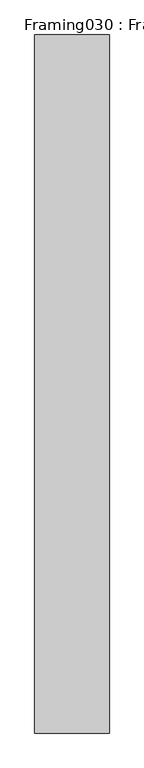
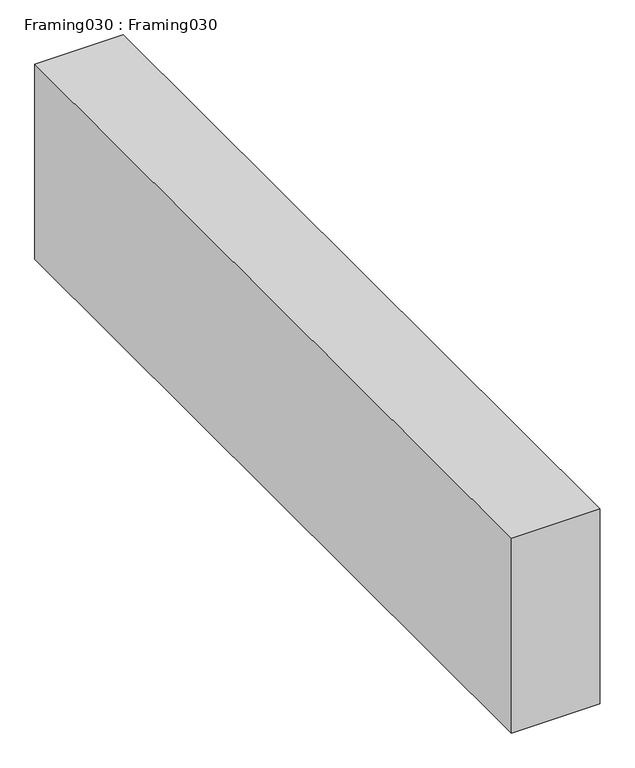
"""IFC4 building model written with IfcOpenShell, lengths in millimetres: proxy geometry, Framing030 : Framing030."""

import ifcopenshell
import ifcopenshell.guid

model = None  # the IFC model being written
_history = None  # IfcOwnerHistory: only IFC2X3 demands one
_inside = {}  # id of a spatial element -> (the spatial element, [elements in it])
_under = {}  # id of a project, library or spatial element -> (it, [spatial elements below it])
_declared = {}  # id of a project -> (the project, [libraries it declares])
_typed = {}  # id of a type object -> (the type object, [elements of that type])
_made_of = {}  # id of a material, layer set ... -> (it, [elements and type objects made of it])


def new_model(schema):
    """Start an empty IFC model of exactly this schema.

    Asked for "IFC4X3", IfcOpenShell would pick the latest addendum, in which some entities
    have other attributes; the version numbers below select the first issue.
    IFC2X3 requires an IfcOwnerHistory on every rooted entity: one is made here for all.
    """
    global model, _history
    if schema == "IFC4X3":
        model = ifcopenshell.file(schema_version=(4, 3, 0, 0))
    else:
        model = ifcopenshell.file(schema=schema)
    _inside.clear()
    _under.clear()
    _declared.clear()
    _typed.clear()
    _made_of.clear()
    _history = None
    if model.schema == "IFC2X3":
        org = make("IfcOrganization", Name="unknown")
        user = make(
            "IfcPersonAndOrganization",
            ThePerson=make("IfcPerson", FamilyName="unknown"),
            TheOrganization=org,
        )
        app = make(
            "IfcApplication",
            ApplicationDeveloper=org,
            Version="unknown",
            ApplicationFullName="unknown",
            ApplicationIdentifier="unknown",
        )
        _history = make(
            "IfcOwnerHistory",
            OwningUser=user,
            OwningApplication=app,
            ChangeAction="ADDED",
            CreationDate=0,
        )
    return model


def make(cls, **values):
    """One entity of the class cls with the attributes given. An attribute that is None is left unset."""
    return model.create_entity(
        cls, **{name: value for name, value in values.items() if value is not None}
    )


def rooted(cls, **values):
    """An entity with a GlobalId (a new one), such as an element, a storey or a relation."""
    return make(cls, GlobalId=ifcopenshell.guid.new(), OwnerHistory=_history, **values)


def si_unit(unit_type, name, prefix=None):
    """IfcSIUnit, for example si_unit("LENGTHUNIT", "METRE", prefix="MILLI")."""
    return make("IfcSIUnit", UnitType=unit_type, Prefix=prefix, Name=name)


def assignment(units):
    """IfcUnitAssignment: the units of a project."""
    return None if units is None else make("IfcUnitAssignment", Units=units)


def point(xyz):
    """IfcCartesianPoint."""
    return None if xyz is None else make("IfcCartesianPoint", Coordinates=xyz)


def direction(xyz):
    """IfcDirection."""
    return None if xyz is None else make("IfcDirection", DirectionRatios=xyz)


def frame(location, z_axis=None, x_axis=None):
    """IfcAxis2Placement3D, a coordinate frame: its origin and axes. An axis left out is left unset."""
    return make(
        "IfcAxis2Placement3D",
        Location=point(location),
        Axis=direction(z_axis),
        RefDirection=direction(x_axis),
    )


def origin():
    """The frame at (0, 0, 0) with its axes left unset."""
    return frame((0.0, 0.0, 0.0))


def place(relative_to, where):
    """IfcLocalPlacement: puts the frame where relative to a parent placement (None: the world)."""
    return make(
        "IfcLocalPlacement", PlacementRelTo=relative_to, RelativePlacement=where
    )


def context(
    kind, dimensions, precision=None, world=None, true_north=None, identifier=None
):
    """IfcGeometricRepresentationContext, for example the 3D "Model" context."""
    return make(
        "IfcGeometricRepresentationContext",
        ContextIdentifier=identifier,
        ContextType=kind,
        CoordinateSpaceDimension=dimensions,
        Precision=precision,
        WorldCoordinateSystem=world,
        TrueNorth=true_north,
    )


def project(units=None, contexts=None):
    """IfcProject with its units and contexts."""
    return rooted(
        "IfcProject",
        Name="project",
        RepresentationContexts=contexts,
        UnitsInContext=assignment(units),
    )


def spatial(cls, under=None, at=None, **own):
    """A site, building, storey or space (cls), placed at a placement, below another one or the project."""
    s = rooted(cls, ObjectPlacement=at, **own)
    if under is not None:
        _under.setdefault(under.id(), (under, []))[1].append(s)
    return s


def polyline(points):
    """IfcPolyline through the points."""
    return make("IfcPolyline", Points=[point(p) for p in points])


def outline(outer, holes=None, kind="AREA"):
    """IfcArbitraryClosedProfileDef: a profile drawn as a closed curve; with holes, ...WithVoids."""
    if holes is None:
        return make("IfcArbitraryClosedProfileDef", ProfileType=kind, OuterCurve=outer)
    return make(
        "IfcArbitraryProfileDefWithVoids",
        ProfileType=kind,
        OuterCurve=outer,
        InnerCurves=holes,
    )


def extrude(swept, where, along, depth):
    """IfcExtrudedAreaSolid: the profile swept, set in the frame where, extruded along a direction by depth."""
    return make(
        "IfcExtrudedAreaSolid",
        SweptArea=swept,
        Position=where,
        ExtrudedDirection=direction(along),
        Depth=depth,
    )


def shape(context_of_items, identifier, shape_type, items):
    """IfcShapeRepresentation: the items that make up one representation, for example the "Body"."""
    return make(
        "IfcShapeRepresentation",
        ContextOfItems=context_of_items,
        RepresentationIdentifier=identifier,
        RepresentationType=shape_type,
        Items=items,
    )


def source(mapping_origin, context_of_items, identifier, shape_type, items):
    """IfcRepresentationMap: a shape defined once, which mapped items show again and again."""
    return make(
        "IfcRepresentationMap",
        MappingOrigin=mapping_origin,
        MappedRepresentation=shape(context_of_items, identifier, shape_type, items),
    )


def transform(
    local_origin,
    x_axis=None,
    y_axis=None,
    z_axis=None,
    scale=None,
    scale2=None,
    scale3=None,
    uniform=True,
):
    """IfcCartesianTransformationOperator3D, or its non-uniform kind. x_axis, y_axis, z_axis: its Axis1, 2, 3."""
    if uniform:
        return make(
            "IfcCartesianTransformationOperator3D",
            Axis1=direction(x_axis),
            Axis2=direction(y_axis),
            LocalOrigin=point(local_origin),
            Scale=scale,
            Axis3=direction(z_axis),
        )
    return make(
        "IfcCartesianTransformationOperator3DnonUniform",
        Axis1=direction(x_axis),
        Axis2=direction(y_axis),
        LocalOrigin=point(local_origin),
        Scale=scale,
        Axis3=direction(z_axis),
        Scale2=scale2,
        Scale3=scale3,
    )


def mapped(mapping_source, mapping_target):
    """IfcMappedItem: shows the shape of a source again, moved by a transform."""
    return make(
        "IfcMappedItem", MappingSource=mapping_source, MappingTarget=mapping_target
    )


def made_of(thing, what):
    """Note that an element or type object is made of a material, layer set ...; save() writes the relation."""
    if what is not None:
        _made_of.setdefault(what.id(), (what, []))[1].append(thing)
    return thing


def element(
    cls,
    number,
    at=None,
    inside=None,
    cuts=None,
    type_object=None,
    material=None,
    context=None,
    identifier="Body",
    shape_type=None,
    held_by="IfcProductDefinitionShape",
    body=None,
    shapes=None,
    **own,
):
    """One element of the class cls, such as IfcWall. Its Tag is "e" and its number.

    at: its placement. inside: the storey or other place that contains it. cuts: it is an
    opening in that element (IfcRelVoidsElement). A single representation is given by context,
    identifier, shape_type and body (its items); several are given by shapes. held_by: the class
    of the entity that holds the representations. save() writes the other relations.
    """
    e = rooted(cls, Tag="e%d" % number, ObjectPlacement=at, **own)
    if body is not None:
        shapes = [shape(context, identifier, shape_type, body)]
    if shapes is not None:
        e.Representation = make(held_by, Representations=shapes)
    if inside is not None:
        _inside.setdefault(inside.id(), (inside, []))[1].append(e)
    if cuts is not None:
        rooted(
            "IfcRelVoidsElement", RelatingBuildingElement=cuts, RelatedOpeningElement=e
        )
    if type_object is not None:
        _typed.setdefault(type_object.id(), (type_object, []))[1].append(e)
    return made_of(e, material)


def aggregate(whole, parts):
    """IfcRelAggregates: a whole, such as a stair, and the parts it consists of."""
    return rooted("IfcRelAggregates", RelatingObject=whole, RelatedObjects=parts)


def save(model, path):
    """Write the relations noted so far, then the file.

    IfcRelAggregates (storeys below a building ...), IfcRelContainedInSpatialStructure (elements
    in a storey), IfcRelDefinesByType, IfcRelAssociatesMaterial and IfcRelDeclares: one each for
    every whole, place, type object, material and project.
    """
    for whole, parts in _under.values():
        aggregate(whole, parts)
    for where, things in _inside.values():
        rooted(
            "IfcRelContainedInSpatialStructure",
            RelatedElements=things,
            RelatingStructure=where,
        )
    for kind, things in _typed.values():
        rooted("IfcRelDefinesByType", RelatedObjects=things, RelatingType=kind)
    for what, things in _made_of.values():
        rooted("IfcRelAssociatesMaterial", RelatedObjects=things, RelatingMaterial=what)
    for by, libraries in _declared.values():
        rooted("IfcRelDeclares", RelatingContext=by, RelatedDefinitions=libraries)
    model.write(path)


def framing030_framing030_16373240(model_context):
    return source(origin(), model_context, "Body", "SweptSolid", [
        extrude(outline(polyline([(13687.8178845, -2827.7925368), (13687.8178845, -4253.3675368), (13535.4178845, -4253.3675368), (13535.4178845, -2827.7925368), (13687.8178845, -2827.7925368)])), frame((0.0, 0.0, 39757.096), z_axis=(0.0, 0.0, 1.0), x_axis=(1.0, 0.0, 0.0)), (0.0, 0.0, 1.0), 355.6),
    ])


if __name__ == "__main__":
    model = new_model("IFC4")
    model_context = context("Model", 3, world=origin())
    ifc_project = project(units=[si_unit("LENGTHUNIT", "METRE", prefix="MILLI")], contexts=[model_context])
    site = spatial("IfcSite", under=ifc_project)
    building = spatial("IfcBuilding", under=site)
    placement = place(None, origin())
    framing030_framing030_shape = framing030_framing030_16373240(model_context)
    element("IfcBuildingElementProxy", 1, Name="Framing030 : Framing030", ObjectType="Framing030 : Framing030", at=placement, inside=building, context=model_context, shape_type="MappedRepresentation", body=[
        mapped(framing030_framing030_shape, transform((0.0, 0.0, 0.0), x_axis=(1.0, 0.0, 0.0), y_axis=(0.0, 1.0, 0.0), z_axis=(0.0, 0.0, 1.0))),
    ])
    save(model, "model.ifc")

# Revit data of these elements
# Type "Framing030 : Framing030"
#   NameOverride = "Framing030"
# Element 1 (IfcBuildingElementProxy, "Framing030 : Framing030")
#   Materials on its faces: "WOOD FRAMING (SEE STRUCT DWGS)"
# Materials
#   "WOOD FRAMING (SEE STRUCT DWGS)": class "Unassigned", colour RGB 224 188 168, transparency 0, Cost = 0
